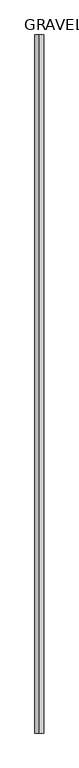
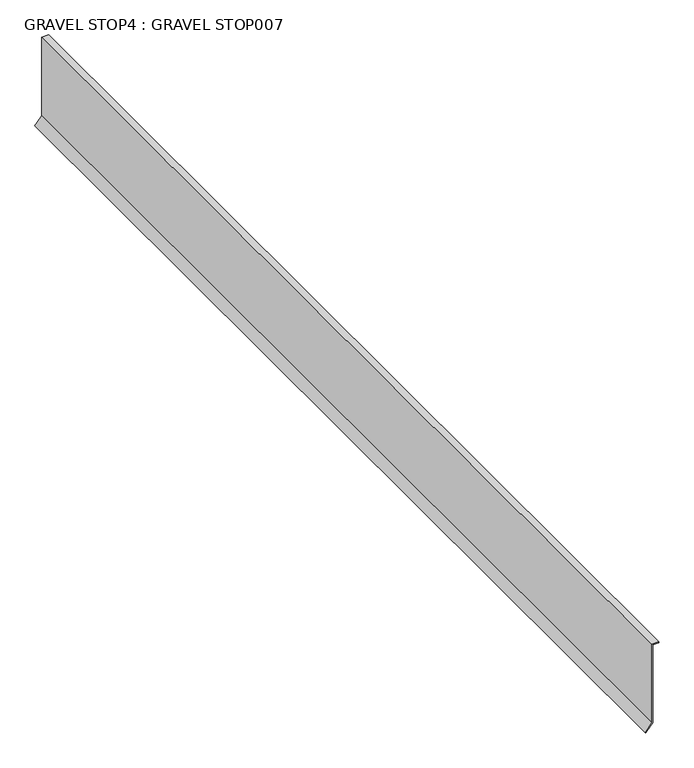
"""IFC4 building model written with IfcOpenShell, lengths in millimetres: proxy geometry, GRAVEL STOP4 : GRAVEL STOP007."""

from ifc_helpers import new_model, si_unit, frame, origin, place, context, project, spatial, polyline, outline, extrude, source, transform, mapped, element, save


def gravel_stop4_gravel_stop007_a1fe0a36(model_context):
    return source(origin(), model_context, "Body", "SweptSolid", [
        extrude(outline(polyline([(40082.2407116, -2815.6343429), (40081.3605882, -2814.5313394), (40097.4918556, -2801.659661), (40253.3245993, -2801.659661), (40253.3245993, -2789.8917422), (40254.7357103, -2789.8917422), (40254.7357103, -2803.070772), (40097.9858473, -2803.070772), (40082.2407116, -2815.6343429)])), frame((0.0, 999.75, 0.0), z_axis=(0.0, 1.0, 0.0), x_axis=(0.0, 0.0, 1.0)), (0.0, 0.0, 1.0), 2000.25),
    ])


if __name__ == "__main__":
    model = new_model("IFC4")
    model_context = context("Model", 3, world=origin())
    ifc_project = project(units=[si_unit("LENGTHUNIT", "METRE", prefix="MILLI")], contexts=[model_context])
    site = spatial("IfcSite", under=ifc_project)
    building = spatial("IfcBuilding", under=site)
    placement = place(None, origin())
    gravel_stop4_gravel_stop007_shape = gravel_stop4_gravel_stop007_a1fe0a36(model_context)
    element("IfcBuildingElementProxy", 1, Name="GRAVEL STOP4 : GRAVEL STOP007", ObjectType="GRAVEL STOP4 : GRAVEL STOP007", at=placement, inside=building, context=model_context, shape_type="MappedRepresentation", body=[
        mapped(gravel_stop4_gravel_stop007_shape, transform((0.0, 0.0, 0.0), x_axis=(1.0, 0.0, 0.0), y_axis=(0.0, 1.0, 0.0), z_axis=(0.0, 0.0, 1.0))),
    ])
    save(model, "model.ifc")

# Revit data of these elements
# Type "GRAVEL STOP4 : GRAVEL STOP007"
#   NameOverride = "GRAVEL STOP007"
# Element 1 (IfcBuildingElementProxy, "GRAVEL STOP4 : GRAVEL STOP007")
#   Materials on its faces: "GRAVEL STOP REQUIRED WITH GRAVEL SURFACE SYSTEMS"
# Materials
#   "GRAVEL STOP REQUIRED WITH GRAVEL SURFACE SYSTEMS": class "Unassigned", colour RGB 170 170 127, transparency 0, Cost = 0
